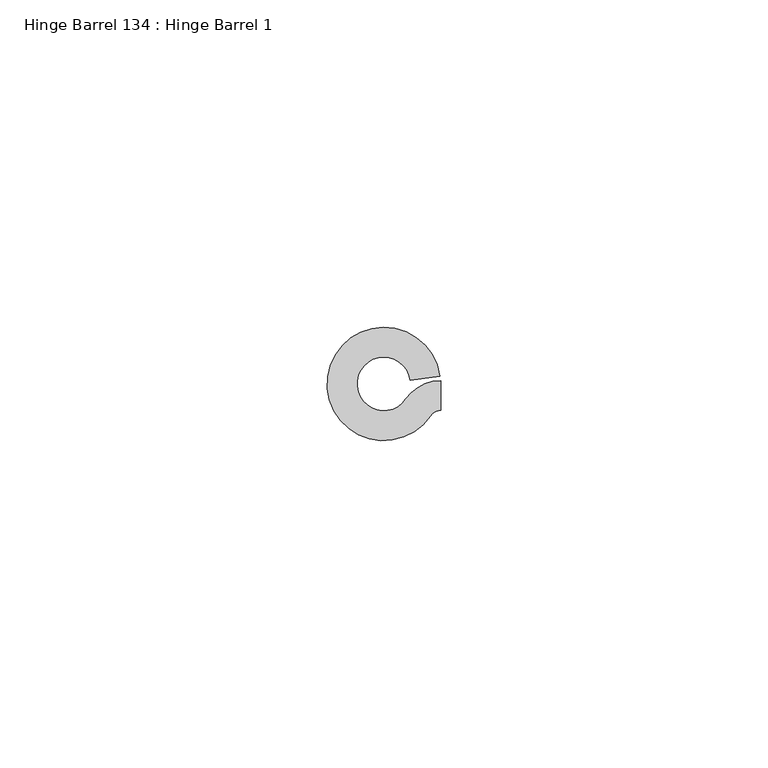
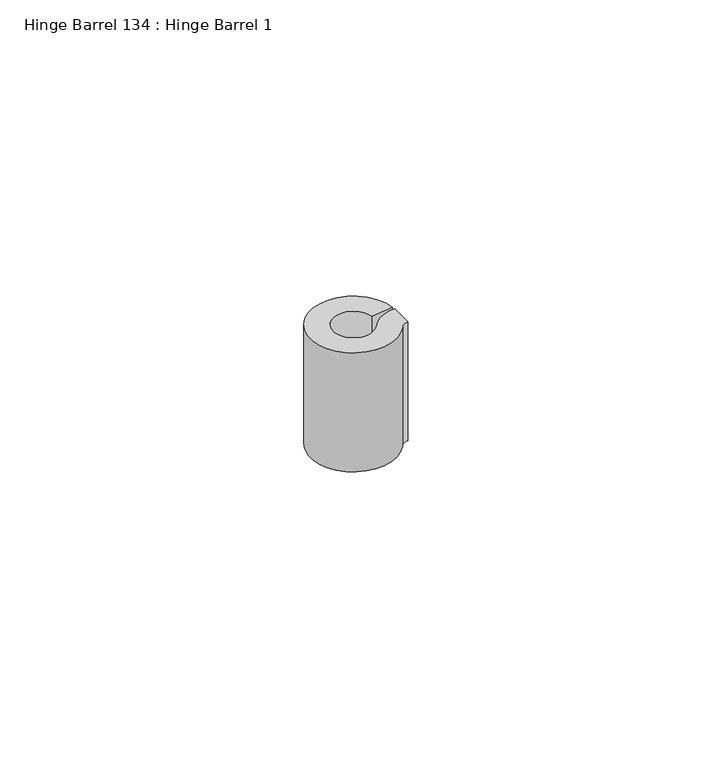
"""IFC4 building model written with IfcOpenShell, lengths in millimetres: proxy geometry, Hinge Barrel 134 : Hinge Barrel 1."""

from ifc_helpers import new_model, si_unit, point, frame, frame_2d, origin, place, context, project, spatial, polyline, circle_curve, trimmed, segment, composite_curve, outline, extrude, source, transform, mapped, element, save


def hinge_barrel_134_hinge_barrel_1_ef8cf91d(model_context):
    return source(origin(), model_context, "Body", "SweptSolid", [
        extrude(outline(composite_curve([segment(trimmed(circle_curve(frame_2d((587327.8245257, -536316.2443067)), 6.4044851), [point((587322.5194669, -536312.6563017))], [point((587327.8245257, -536309.8398216))], False, "CARTESIAN"), True, "CONTINUOUS"), segment(polyline([(587327.8245257, -536309.8398216), (587327.8245257, -536314.4038841)]), True, "CONTINUOUS"), segment(trimmed(circle_curve(frame_2d((587327.8245257, -536316.2443067)), 1.8404226), [point((587327.8245257, -536314.4038841))], [point((587326.3000393, -536315.2132409))], True, "CARTESIAN"), True, "CONTINUOUS"), segment(trimmed(circle_curve(frame_2d((587319.1320739, -536310.3652841)), 8.6534625), [point((587326.3000393, -536315.2132409))], [point((587327.7022899, -536309.1678654))], False, "CARTESIAN"), True, "CONTINUOUS"), segment(polyline([(587327.7022899, -536309.1678654), (587323.1821338, -536309.7994153)]), True, "CONTINUOUS"), segment(trimmed(circle_curve(frame_2d((587319.1320739, -536310.3652841)), 4.0894), [point((587323.1821338, -536309.7994153))], [point((587322.5194669, -536312.6563017))], True, "CARTESIAN"), True, "CONTINUOUS")], self_intersect=False)), frame((0.0, 0.0, 1962.15), z_axis=(0.0, 0.0, 1.0), x_axis=(1.0, 0.0, 0.0)), (0.0, 0.0, 1.0), 25.4),
    ])


if __name__ == "__main__":
    model = new_model("IFC4")
    model_context = context("Model", 3, world=origin())
    ifc_project = project(units=[si_unit("LENGTHUNIT", "METRE", prefix="MILLI")], contexts=[model_context])
    site = spatial("IfcSite", under=ifc_project)
    building = spatial("IfcBuilding", under=site)
    placement = place(None, origin())
    hinge_barrel_134_hinge_barrel_1_shape = hinge_barrel_134_hinge_barrel_1_ef8cf91d(model_context)
    element("IfcBuildingElementProxy", 1, Name="Hinge Barrel 134 : Hinge Barrel 1", ObjectType="Hinge Barrel 134 : Hinge Barrel 1", at=placement, inside=building, context=model_context, shape_type="MappedRepresentation", body=[
        mapped(hinge_barrel_134_hinge_barrel_1_shape, transform((0.0, 0.0, 0.0), x_axis=(1.0, 0.0, 0.0), y_axis=(0.0, 1.0, 0.0), z_axis=(0.0, 0.0, 1.0))),
    ])
    save(model, "model.ifc")

# Revit data of these elements
# Element 1 (IfcBuildingElementProxy, "Hinge Barrel 134 : Hinge Barrel 1")
#   Materials on its faces: "6\"X6\" WELD-ON STL BUTT HINGE"
# Materials
#   "6\"X6\" WELD-ON STL BUTT HINGE": class "Metal", colour RGB 189 187 185, transparency 0, Description = "Carbon steel", Cost = 0
